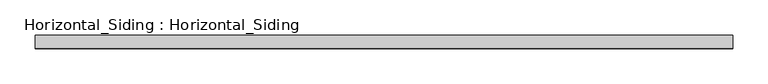
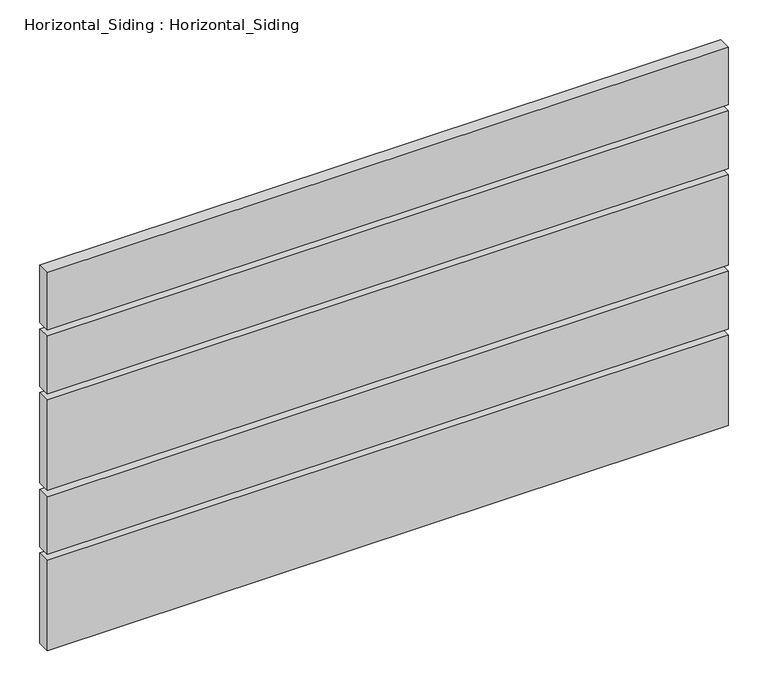
"""IFC4 building model written with IfcOpenShell, lengths in millimetres: plate geometry, Horizontal_Siding : Horizontal_Siding."""

from ifc_helpers import new_model, si_unit, frame, origin, place, context, project, spatial, polyline, outline, extrude, source, transform, mapped, element, save


def horizontal_siding_horizontal_siding_405d1c8b(model_context):
    return source(origin(), model_context, "Body", "SweptSolid", [
        extrude(outline(polyline([(497.0011771, -19.05), (-497.0011771, -19.05), (-497.0011771, 0.0), (497.0011771, 0.0), (497.0011771, -19.05)])), frame((0.0, 0.0, 9.525), z_axis=(0.0, 0.0, 1.0), x_axis=(1.0, 0.0, 0.0)), (0.0, 0.0, 1.0), 139.7),
        extrude(outline(polyline([(497.0011771, -19.05), (-497.0011771, -19.05), (-497.0011771, 0.0), (497.0011771, 0.0), (497.0011771, -19.05)])), frame((0.0, 0.0, 158.75), z_axis=(0.0, 0.0, 1.0), x_axis=(1.0, 0.0, 0.0)), (0.0, 0.0, 1.0), 88.9),
        extrude(outline(polyline([(497.0011771, -19.05), (-497.0011771, -19.05), (-497.0011771, 0.0), (497.0011771, 0.0), (497.0011771, -19.05)])), frame((0.0, 0.0, 257.175), z_axis=(0.0, 0.0, 1.0), x_axis=(1.0, 0.0, 0.0)), (0.0, 0.0, 1.0), 139.7),
        extrude(outline(polyline([(497.0011771, -19.05), (-497.0011771, -19.05), (-497.0011771, 0.0), (497.0011771, 0.0), (497.0011771, -19.05)])), frame((0.0, 0.0, 406.4), z_axis=(0.0, 0.0, 1.0), x_axis=(1.0, 0.0, 0.0)), (0.0, 0.0, 1.0), 88.9),
        extrude(outline(polyline([(497.0011771, -19.05), (-497.0011771, -19.05), (-497.0011771, 0.0), (497.0011771, 0.0), (497.0011771, -19.05)])), frame((0.0, 0.0, 504.825), z_axis=(0.0, 0.0, 1.0), x_axis=(1.0, 0.0, 0.0)), (0.0, 0.0, 1.0), 88.9),
    ])


if __name__ == "__main__":
    model = new_model("IFC4")
    model_context = context("Model", 3, world=origin())
    ifc_project = project(units=[si_unit("LENGTHUNIT", "METRE", prefix="MILLI")], contexts=[model_context])
    site = spatial("IfcSite", under=ifc_project)
    building = spatial("IfcBuilding", under=site)
    placement = place(None, origin())
    horizontal_siding_horizontal_siding_shape = horizontal_siding_horizontal_siding_405d1c8b(model_context)
    element("IfcPlate", 1, ObjectType="Horizontal_Siding : Horizontal_Siding", at=placement, inside=building, context=model_context, shape_type="MappedRepresentation", body=[
        mapped(horizontal_siding_horizontal_siding_shape, transform((0.0, 0.0, 0.0), x_axis=(1.0, 0.0, 0.0), y_axis=(0.0, 1.0, 0.0), z_axis=(0.0, 0.0, 1.0))),
    ])
    save(model, "model.ifc")

# Revit data of these elements
# Type "Horizontal_Siding : Horizontal_Siding"
#   Type Mark = "OUT"
#   Analytic Construction = "<None>"
#   extend = 0' - 2 3/4"
#   Width_2 = 0' - 3 1/2"
#   Width_1 = 0' - 5 1/2"
#   Gap = 0' - 0 3/8"
#   Plank Material = SLOTTED WOOD FENCE (THERMALLY MODIFIED WOOD: ARBOR WOOD)\n(EXTERIOR STAIN : PENOFIN VERDE EXT. STAIN - COLOR: CEDAR)
# Element 1 (IfcPlate, "Horizontal_Siding : Horizontal_Siding")
#   Materials on its faces: "SLOTTED WOOD FENCE (THERMALLY MODIFIED WOOD: ARBOR WOOD)\n(EXTERIOR STAIN : PENOFIN VERDE EXT. STAIN - COLOR: CEDAR)"
# Materials
#   "SLOTTED WOOD FENCE (THERMALLY MODIFIED WOOD: ARBOR WOOD)\n(EXTERIOR STAIN : PENOFIN VERDE EXT. STAIN - COLOR: CEDAR)": class "Wood", colour RGB 164 134 123, transparency 0, Description = "Pinus Echinata", Cost = 0
